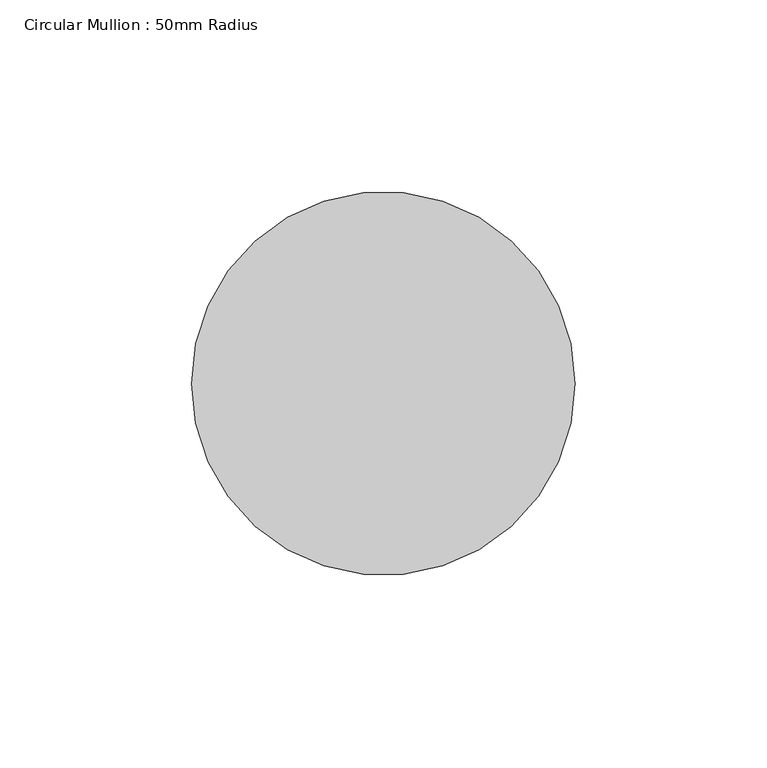
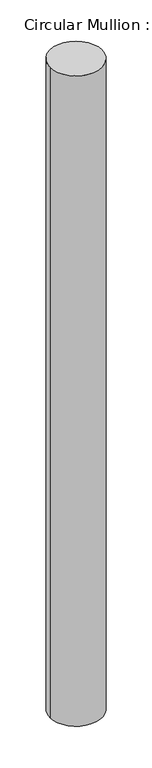
"""IFC4 building model written with IfcOpenShell, lengths in millimetres: member geometry, Circular Mullion : 50mm Radius."""

from ifc_helpers import new_model, si_unit, point, frame, origin, origin_2d, place, context, project, spatial, circle_curve, trimmed, segment, composite_curve, outline, extrude, source, transform, mapped, element, save


def circular_mullion_50mm_radius_d1fe3595(model_context):
    return source(origin(), model_context, "Body", "SweptSolid", [
        extrude(outline(composite_curve([segment(trimmed(circle_curve(origin_2d(), 50.0), [point((50.0, 0.0))], [point((-50.0, 0.0))], False, "CARTESIAN"), True, "CONTINUOUS"), segment(trimmed(circle_curve(origin_2d(), 50.0), [point((-50.0, 0.0))], [point((50.0, 0.0))], False, "CARTESIAN"), True, "CONTINUOUS")], self_intersect=False)), frame((0.0, 0.0, -1313.9108186), z_axis=(0.0, 0.0, 1.0), x_axis=(1.0, 0.0, 0.0)), (0.0, 0.0, 1.0), 1313.9108186),
    ])


if __name__ == "__main__":
    model = new_model("IFC4")
    model_context = context("Model", 3, world=origin())
    ifc_project = project(units=[si_unit("LENGTHUNIT", "METRE", prefix="MILLI")], contexts=[model_context])
    site = spatial("IfcSite", under=ifc_project)
    building = spatial("IfcBuilding", under=site)
    placement = place(None, origin())
    circular_mullion_50mm_radius_shape = circular_mullion_50mm_radius_d1fe3595(model_context)
    element("IfcMember", 1, ObjectType="Circular Mullion : 50mm Radius", at=placement, inside=building, context=model_context, shape_type="MappedRepresentation", body=[
        mapped(circular_mullion_50mm_radius_shape, transform((0.0, 0.0, 0.0), x_axis=(1.0, 0.0, 0.0), y_axis=(0.0, 1.0, 0.0), z_axis=(0.0, 0.0, 1.0))),
    ])
    save(model, "model.ifc")

# Revit data of these elements
# Type "Circular Mullion : 50mm Radius"
#   built-in parameter 1007350 = 0.164042 (stored number, unit not read)
# Element 1 (IfcMember, "Circular Mullion : 50mm Radius")
#   Materials on its faces: "Aluminium"
# Materials
#   "Aluminium": class "Metal", colour RGB 247 247 247, transparency 0, Description = "Aluminium 6061", Cost = 0
